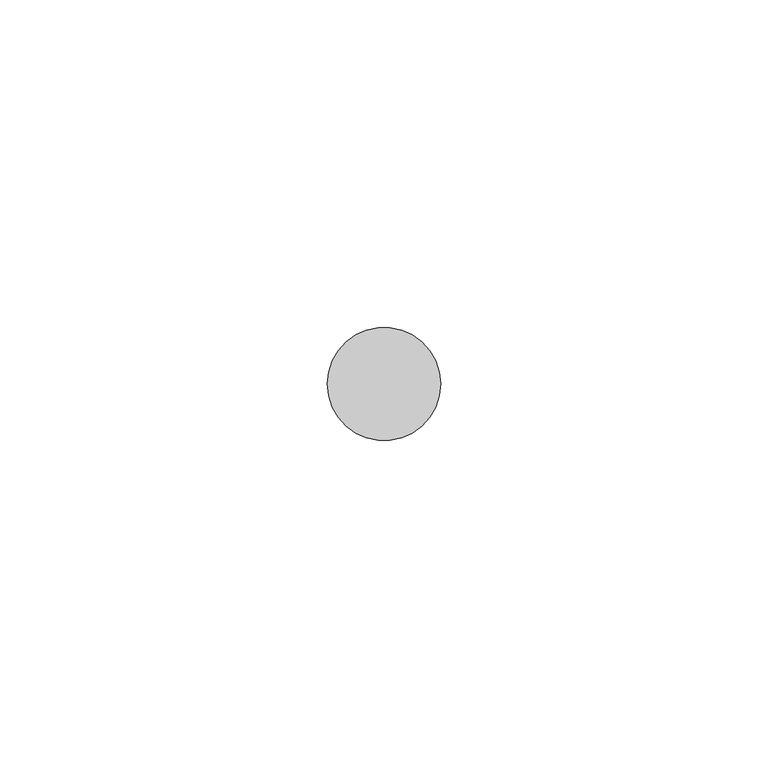
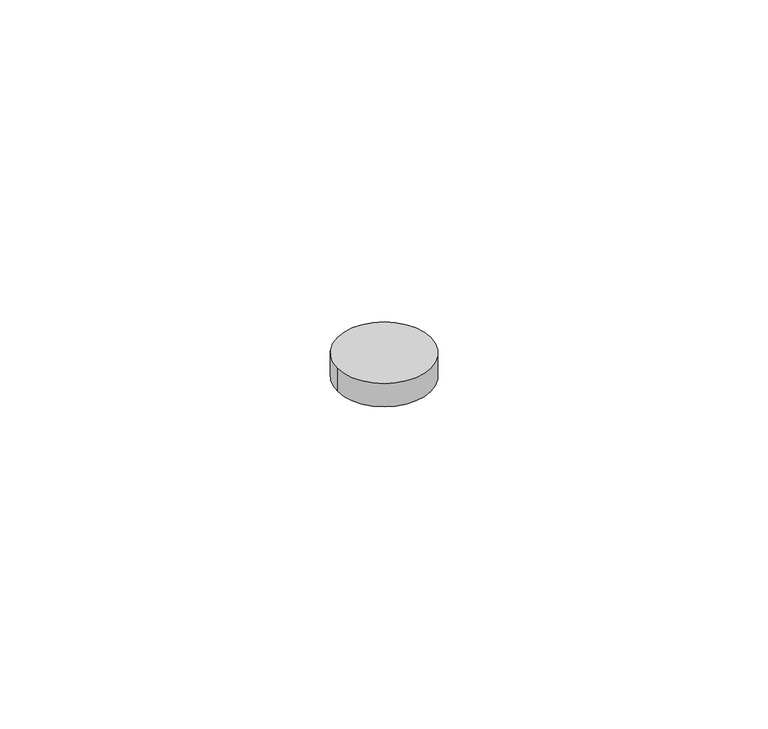
"""IFC4 building model written with IfcOpenShell, lengths in millimetres: proxy geometry, Hinge Pin Keeper6 : Hinge Pin Keeper."""

from ifc_helpers import new_model, si_unit, point, frame, frame_2d, origin, place, context, project, spatial, circle_curve, trimmed, segment, composite_curve, outline, extrude, source, transform, mapped, element, save


def generic_models_5ab26af4(model_context):
    return source(origin(), model_context, "Body", "SweptSolid", [
        extrude(outline(composite_curve([segment(trimmed(circle_curve(frame_2d((587319.1320739, -534100.7049841)), 8.6534625), [point((587310.4786114, -534100.7049841))], [point((587327.7855364, -534100.7049841))], False, "CARTESIAN"), True, "CONTINUOUS"), segment(trimmed(circle_curve(frame_2d((587319.1320739, -534100.7049841)), 8.6534625), [point((587327.7855364, -534100.7049841))], [point((587310.4786114, -534100.7049841))], False, "CARTESIAN"), True, "CONTINUOUS")], self_intersect=False)), frame((0.0, 0.0, 458.9859375), z_axis=(0.0, 0.0, 1.0), x_axis=(1.0, 0.0, 0.0)), (0.0, 0.0, 1.0), 4.5640625),
    ])


if __name__ == "__main__":
    model = new_model("IFC4")
    model_context = context("Model", 3, world=origin())
    ifc_project = project(units=[si_unit("LENGTHUNIT", "METRE", prefix="MILLI")], contexts=[model_context])
    site = spatial("IfcSite", under=ifc_project)
    building = spatial("IfcBuilding", under=site)
    placement = place(None, origin())
    generic_models_shape = generic_models_5ab26af4(model_context)
    element("IfcBuildingElementProxy", 1, Name="Hinge Pin Keeper6 : Hinge Pin Keeper", ObjectType="Hinge Pin Keeper6 : Hinge Pin Keeper", at=placement, inside=building, context=model_context, shape_type="MappedRepresentation", body=[
        mapped(generic_models_shape, transform((0.0, 0.0, 0.0), x_axis=(1.0, 0.0, 0.0), y_axis=(0.0, 1.0, 0.0), z_axis=(0.0, 0.0, 1.0))),
    ])
    save(model, "model.ifc")

# Revit data of these elements
# Element 1 (IfcBuildingElementProxy, "Hinge Pin Keeper6 : Hinge Pin Keeper")
#   Materials on its faces: "6\"X6\" WELD-ON STL BUTT HINGE"
# Materials
#   "6\"X6\" WELD-ON STL BUTT HINGE": class "Metal", colour RGB 189 187 185, transparency 0, Description = "Carbon steel", Cost = 0
